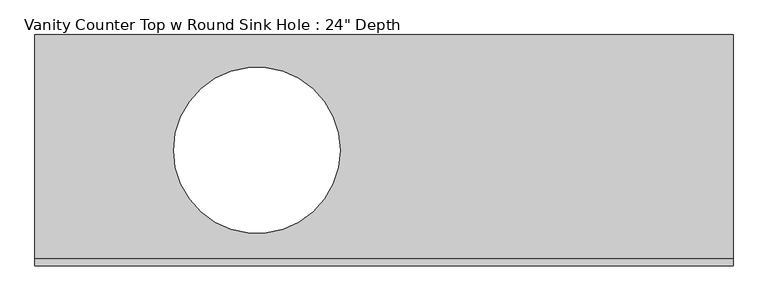
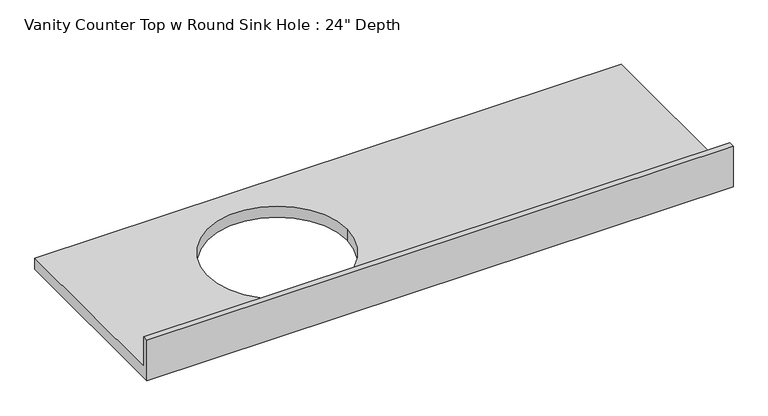
"""IFC4 building model written with IfcOpenShell, lengths in millimetres: furniture geometry."""

from ifc_helpers import new_model, si_unit, frame, origin, place, context, project, spatial, polyline, circle_curve, source, transform, mapped, element, save
from ifc_brep_helpers import plane_surface, revolved_surface, advanced_brep


def furniture_cfdb0dcc(model_context):
    return source(origin(), model_context, "Body", "AdvancedBrep", [
        advanced_brep(
        [(-1327.4622951, 635.0, 787.4), (-1327.4622951, 19.05, 787.4), (590.2377049, 19.05, 787.4), (590.2377049, 635.0, 787.4), (-489.2622951, 317.5, 787.4), (-946.4622951, 317.5, 787.4), (590.2377049, 0.0, 749.3), (-1327.4622951, 0.0, 749.3), (-1327.4622951, 635.0, 749.3), (590.2377049, 635.0, 749.3), (-946.4622951, 317.5, 749.3), (-489.2622951, 317.5, 749.3), (590.2377049, 0.0, 889.0), (-1327.4622951, 0.0, 889.0), (-1327.4622951, 19.05, 889.0), (590.2377049, 19.05, 889.0)],
        [
            (0, 1),
            (1, 2),
            (2, 3),
            (3, 0),
            (4, 5, circle_curve(frame((-717.8622951, 317.5, 787.4), z_axis=(0.0, 0.0, -1.0), x_axis=(1.0, 0.0, 0.0)), 228.6)),
            (5, 4, circle_curve(frame((-717.8622951, 317.5, 787.4), z_axis=(0.0, 0.0, -1.0), x_axis=(1.0, 0.0, 0.0)), 228.6)),
            (6, 7),
            (7, 8),
            (8, 9),
            (9, 6),
            (10, 11, circle_curve(frame((-717.8622951, 317.5, 749.3), z_axis=(0.0, 0.0, 1.0), x_axis=(1.0, 0.0, 0.0)), 228.6)),
            (11, 10, circle_curve(frame((-717.8622951, 317.5, 749.3), z_axis=(0.0, 0.0, 1.0), x_axis=(1.0, 0.0, 0.0)), 228.6)),
            (6, 12),
            (12, 13),
            (13, 7),
            (13, 14),
            (14, 1),
            (0, 8),
            (3, 9),
            (2, 15),
            (15, 12),
            (15, 14),
            (5, 10),
            (11, 4),
        ],
        [
            plane_surface(frame((-1327.4622951, 0.0, 787.4), z_axis=(0.0, 0.0, 1.0), x_axis=(-1.0, 0.0, 0.0))),
            plane_surface(frame((-1327.4622951, 0.0, 749.3), z_axis=(0.0, 0.0, -1.0), x_axis=(1.0, 0.0, 0.0))),
            plane_surface(frame((590.2377049, 0.0, 787.4), z_axis=(0.0, -1.0, 0.0), x_axis=(0.0, 0.0, -1.0))),
            plane_surface(frame((-1327.4622951, 0.0, 787.4), z_axis=(-1.0, 0.0, 0.0), x_axis=(0.0, 0.0, -1.0))),
            plane_surface(frame((-1327.4622951, 635.0, 787.4), z_axis=(0.0, 1.0, 0.0), x_axis=(0.0, 0.0, -1.0))),
            plane_surface(frame((590.2377049, 635.0, 787.4), z_axis=(1.0, 0.0, 0.0), x_axis=(0.0, 0.0, -1.0))),
            plane_surface(frame((-1327.4622951, 0.0, 889.0), z_axis=(0.0, 0.0, 1.0), x_axis=(0.0, 1.0, 0.0))),
            plane_surface(frame((-1327.4622951, 19.05, 889.0), z_axis=(0.0, 1.0, 0.0), x_axis=(0.0, 0.0, -1.0))),
            revolved_surface(polyline([(-489.26229509999996, 317.5, 787.4), (-489.26229509999996, 317.5, 749.3)]), (-717.8622951, 317.5, 749.3), (0.0, 0.0, 1.0)),
        ],
        [
            (0, [[1, 2, 3, 4], [5, 6]]),
            (1, [[7, 8, 9, 10], [11, 12]]),
            (2, [[13, 14, 15, -7]]),
            (3, [[-15, 16, 17, -1, 18, -8]]),
            (4, [[19, -9, -18, -4]]),
            (5, [[-19, -3, 20, 21, -13, -10]]),
            (6, [[-14, -21, 22, -16]]),
            (7, [[-20, -2, -17, -22]]),
            (8, [[-6, 23, -12, 24]]),
            (8, [[-11, -23, -5, -24]]),
        ],
    ),
    ])


if __name__ == "__main__":
    model = new_model("IFC4")
    model_context = context("Model", 3, world=origin())
    ifc_project = project(units=[si_unit("LENGTHUNIT", "METRE", prefix="MILLI")], contexts=[model_context])
    site = spatial("IfcSite", under=ifc_project)
    building = spatial("IfcBuilding", under=site)
    placement = place(None, origin())
    furniture_shape = furniture_cfdb0dcc(model_context)
    element("IfcFurniture", 1, ObjectType="Vanity Counter Top w Round Sink Hole : 24\" Depth", at=placement, inside=building, context=model_context, shape_type="MappedRepresentation", body=[
        mapped(furniture_shape, transform((0.0, 0.0, 0.0), x_axis=(1.0, 0.0, 0.0), y_axis=(0.0, 1.0, 0.0), z_axis=(0.0, 0.0, 1.0))),
    ])
    save(model, "model.ifc")

# Revit data of these elements
# Type "Vanity Counter Top w Round Sink Hole : 24\" Depth"
#   Assembly Code = "C1030400"
#   Counter Thickness = 0' - 1 1/2"
#   Depth = 2' - 1"
#   Height = 2' - 7"
#   Length [instance default] = 4' - 0"
#   Sink Location [instance default] = 2' - 0"
#   Sink Location To Wall [instance default] = 0' - 4"
#   Sink Opening Width [instance default] = 1' - 5"
#   Counter Top Material = Laminate, Blue, Matte
#   Default Elevation = 0
# Element 1 (IfcFurniture, "Vanity Counter Top w Round Sink Hole : 24\" Depth")
#   Length = 6' - 3 1/2"
#   Materials on its faces: "Laminate, Blue, Matte"
# Materials
#   "Laminate, Blue, Matte": class "Plastic", colour RGB 85 101 155, transparency 0, Description = "Plastic Laminate - Blue, Matte", Cost = 0
